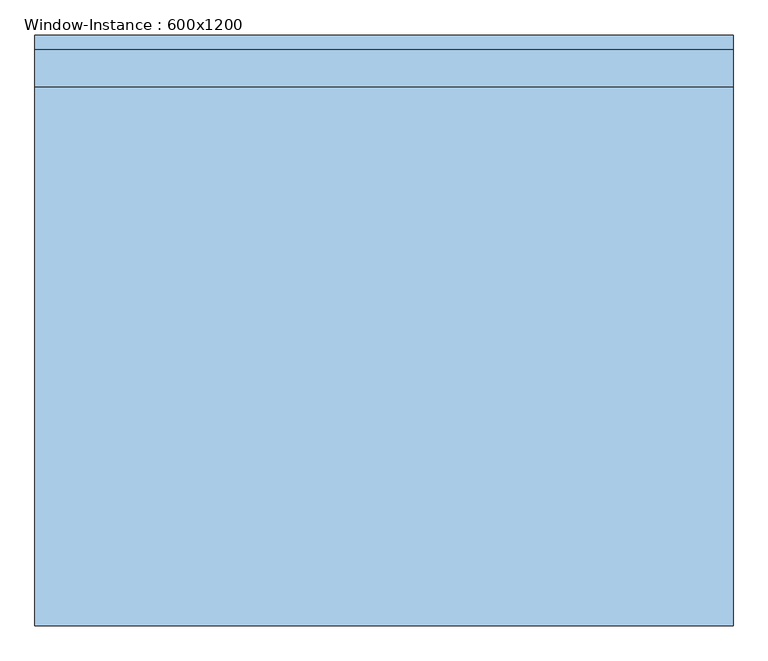
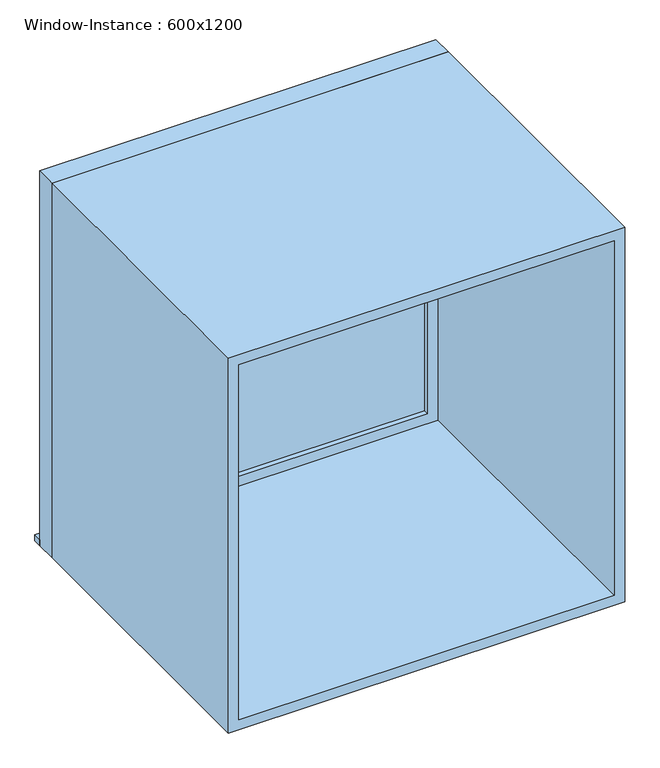
"""IFC4 building model written with IfcOpenShell, lengths in millimetres: window geometry, Window-Instance : 600x1200."""

import ifcopenshell
import ifcopenshell.guid

model = None  # the IFC model being written
_history = None  # IfcOwnerHistory: only IFC2X3 demands one
_inside = {}  # id of a spatial element -> (the spatial element, [elements in it])
_under = {}  # id of a project, library or spatial element -> (it, [spatial elements below it])
_declared = {}  # id of a project -> (the project, [libraries it declares])
_typed = {}  # id of a type object -> (the type object, [elements of that type])
_made_of = {}  # id of a material, layer set ... -> (it, [elements and type objects made of it])


def new_model(schema):
    """Start an empty IFC model of exactly this schema.

    Asked for "IFC4X3", IfcOpenShell would pick the latest addendum, in which some entities
    have other attributes; the version numbers below select the first issue.
    IFC2X3 requires an IfcOwnerHistory on every rooted entity: one is made here for all.
    """
    global model, _history
    if schema == "IFC4X3":
        model = ifcopenshell.file(schema_version=(4, 3, 0, 0))
    else:
        model = ifcopenshell.file(schema=schema)
    _inside.clear()
    _under.clear()
    _declared.clear()
    _typed.clear()
    _made_of.clear()
    _history = None
    if model.schema == "IFC2X3":
        org = make("IfcOrganization", Name="unknown")
        user = make(
            "IfcPersonAndOrganization",
            ThePerson=make("IfcPerson", FamilyName="unknown"),
            TheOrganization=org,
        )
        app = make(
            "IfcApplication",
            ApplicationDeveloper=org,
            Version="unknown",
            ApplicationFullName="unknown",
            ApplicationIdentifier="unknown",
        )
        _history = make(
            "IfcOwnerHistory",
            OwningUser=user,
            OwningApplication=app,
            ChangeAction="ADDED",
            CreationDate=0,
        )
    return model


def make(cls, **values):
    """One entity of the class cls with the attributes given. An attribute that is None is left unset."""
    return model.create_entity(
        cls, **{name: value for name, value in values.items() if value is not None}
    )


def rooted(cls, **values):
    """An entity with a GlobalId (a new one), such as an element, a storey or a relation."""
    return make(cls, GlobalId=ifcopenshell.guid.new(), OwnerHistory=_history, **values)


def si_unit(unit_type, name, prefix=None):
    """IfcSIUnit, for example si_unit("LENGTHUNIT", "METRE", prefix="MILLI")."""
    return make("IfcSIUnit", UnitType=unit_type, Prefix=prefix, Name=name)


def assignment(units):
    """IfcUnitAssignment: the units of a project."""
    return None if units is None else make("IfcUnitAssignment", Units=units)


def point(xyz):
    """IfcCartesianPoint."""
    return None if xyz is None else make("IfcCartesianPoint", Coordinates=xyz)


def direction(xyz):
    """IfcDirection."""
    return None if xyz is None else make("IfcDirection", DirectionRatios=xyz)


def frame(location, z_axis=None, x_axis=None):
    """IfcAxis2Placement3D, a coordinate frame: its origin and axes. An axis left out is left unset."""
    return make(
        "IfcAxis2Placement3D",
        Location=point(location),
        Axis=direction(z_axis),
        RefDirection=direction(x_axis),
    )


def origin():
    """The frame at (0, 0, 0) with its axes left unset."""
    return frame((0.0, 0.0, 0.0))


def place(relative_to, where):
    """IfcLocalPlacement: puts the frame where relative to a parent placement (None: the world)."""
    return make(
        "IfcLocalPlacement", PlacementRelTo=relative_to, RelativePlacement=where
    )


def context(
    kind, dimensions, precision=None, world=None, true_north=None, identifier=None
):
    """IfcGeometricRepresentationContext, for example the 3D "Model" context."""
    return make(
        "IfcGeometricRepresentationContext",
        ContextIdentifier=identifier,
        ContextType=kind,
        CoordinateSpaceDimension=dimensions,
        Precision=precision,
        WorldCoordinateSystem=world,
        TrueNorth=true_north,
    )


def project(units=None, contexts=None):
    """IfcProject with its units and contexts."""
    return rooted(
        "IfcProject",
        Name="project",
        RepresentationContexts=contexts,
        UnitsInContext=assignment(units),
    )


def spatial(cls, under=None, at=None, **own):
    """A site, building, storey or space (cls), placed at a placement, below another one or the project."""
    s = rooted(cls, ObjectPlacement=at, **own)
    if under is not None:
        _under.setdefault(under.id(), (under, []))[1].append(s)
    return s


def polyline(points):
    """IfcPolyline through the points."""
    return make("IfcPolyline", Points=[point(p) for p in points])


def outline(outer, holes=None, kind="AREA"):
    """IfcArbitraryClosedProfileDef: a profile drawn as a closed curve; with holes, ...WithVoids."""
    if holes is None:
        return make("IfcArbitraryClosedProfileDef", ProfileType=kind, OuterCurve=outer)
    return make(
        "IfcArbitraryProfileDefWithVoids",
        ProfileType=kind,
        OuterCurve=outer,
        InnerCurves=holes,
    )


def extrude(swept, where, along, depth):
    """IfcExtrudedAreaSolid: the profile swept, set in the frame where, extruded along a direction by depth."""
    return make(
        "IfcExtrudedAreaSolid",
        SweptArea=swept,
        Position=where,
        ExtrudedDirection=direction(along),
        Depth=depth,
    )


def shape(context_of_items, identifier, shape_type, items):
    """IfcShapeRepresentation: the items that make up one representation, for example the "Body"."""
    return make(
        "IfcShapeRepresentation",
        ContextOfItems=context_of_items,
        RepresentationIdentifier=identifier,
        RepresentationType=shape_type,
        Items=items,
    )


def source(mapping_origin, context_of_items, identifier, shape_type, items):
    """IfcRepresentationMap: a shape defined once, which mapped items show again and again."""
    return make(
        "IfcRepresentationMap",
        MappingOrigin=mapping_origin,
        MappedRepresentation=shape(context_of_items, identifier, shape_type, items),
    )


def transform(
    local_origin,
    x_axis=None,
    y_axis=None,
    z_axis=None,
    scale=None,
    scale2=None,
    scale3=None,
    uniform=True,
):
    """IfcCartesianTransformationOperator3D, or its non-uniform kind. x_axis, y_axis, z_axis: its Axis1, 2, 3."""
    if uniform:
        return make(
            "IfcCartesianTransformationOperator3D",
            Axis1=direction(x_axis),
            Axis2=direction(y_axis),
            LocalOrigin=point(local_origin),
            Scale=scale,
            Axis3=direction(z_axis),
        )
    return make(
        "IfcCartesianTransformationOperator3DnonUniform",
        Axis1=direction(x_axis),
        Axis2=direction(y_axis),
        LocalOrigin=point(local_origin),
        Scale=scale,
        Axis3=direction(z_axis),
        Scale2=scale2,
        Scale3=scale3,
    )


def mapped(mapping_source, mapping_target):
    """IfcMappedItem: shows the shape of a source again, moved by a transform."""
    return make(
        "IfcMappedItem", MappingSource=mapping_source, MappingTarget=mapping_target
    )


def made_of(thing, what):
    """Note that an element or type object is made of a material, layer set ...; save() writes the relation."""
    if what is not None:
        _made_of.setdefault(what.id(), (what, []))[1].append(thing)
    return thing


def element(
    cls,
    number,
    at=None,
    inside=None,
    cuts=None,
    type_object=None,
    material=None,
    context=None,
    identifier="Body",
    shape_type=None,
    held_by="IfcProductDefinitionShape",
    body=None,
    shapes=None,
    **own,
):
    """One element of the class cls, such as IfcWall. Its Tag is "e" and its number.

    at: its placement. inside: the storey or other place that contains it. cuts: it is an
    opening in that element (IfcRelVoidsElement). A single representation is given by context,
    identifier, shape_type and body (its items); several are given by shapes. held_by: the class
    of the entity that holds the representations. save() writes the other relations.
    """
    e = rooted(cls, Tag="e%d" % number, ObjectPlacement=at, **own)
    if body is not None:
        shapes = [shape(context, identifier, shape_type, body)]
    if shapes is not None:
        e.Representation = make(held_by, Representations=shapes)
    if inside is not None:
        _inside.setdefault(inside.id(), (inside, []))[1].append(e)
    if cuts is not None:
        rooted(
            "IfcRelVoidsElement", RelatingBuildingElement=cuts, RelatedOpeningElement=e
        )
    if type_object is not None:
        _typed.setdefault(type_object.id(), (type_object, []))[1].append(e)
    return made_of(e, material)


def aggregate(whole, parts):
    """IfcRelAggregates: a whole, such as a stair, and the parts it consists of."""
    return rooted("IfcRelAggregates", RelatingObject=whole, RelatedObjects=parts)


def save(model, path):
    """Write the relations noted so far, then the file.

    IfcRelAggregates (storeys below a building ...), IfcRelContainedInSpatialStructure (elements
    in a storey), IfcRelDefinesByType, IfcRelAssociatesMaterial and IfcRelDeclares: one each for
    every whole, place, type object, material and project.
    """
    for whole, parts in _under.values():
        aggregate(whole, parts)
    for where, things in _inside.values():
        rooted(
            "IfcRelContainedInSpatialStructure",
            RelatedElements=things,
            RelatingStructure=where,
        )
    for kind, things in _typed.values():
        rooted("IfcRelDefinesByType", RelatedObjects=things, RelatingType=kind)
    for what, things in _made_of.values():
        rooted("IfcRelAssociatesMaterial", RelatedObjects=things, RelatingMaterial=what)
    for by, libraries in _declared.values():
        rooted("IfcRelDeclares", RelatingContext=by, RelatedDefinitions=libraries)
    model.write(path)


def window_instance_600x1200_03e1e92d(model_context):
    return source(origin(), model_context, "Body", "SweptSolid", [
        extrude(outline(polyline([(-638.1, 520.4), (561.9, 520.4), (561.9, 495.0), (-638.1, 495.0), (-638.1, 520.4)])), frame((0.0, 0.0, 900.0), z_axis=(0.0, 0.0, 1.0), x_axis=(1.0, 0.0, 0.0)), (0.0, 0.0, 1.0), 19.05),
        extrude(outline(polyline([(498.4, 446.425), (-574.6, 446.425), (-574.6, 459.125), (498.4, 459.125), (498.4, 446.425)])), frame((0.0, 0.0, 963.5), z_axis=(0.0, 0.0, 1.0), x_axis=(1.0, 0.0, 0.0)), (0.0, 0.0, 1.0), 1073.0),
        extrude(outline(polyline([(2080.95, -619.05), (919.05, -619.05), (919.05, 542.85), (2080.95, 542.85), (2080.95, -619.05)]), holes=[polyline([(2036.5, -574.6), (2036.5, 498.4), (963.5, 498.4), (963.5, -574.6), (2036.5, -574.6)])]), frame((0.0, 430.55, 0.0), z_axis=(0.0, 1.0, 0.0), x_axis=(0.0, 0.0, 1.0)), (0.0, 0.0, 1.0), 44.45),
        extrude(outline(polyline([(2100.0, -638.1), (900.0, -638.1), (900.0, 561.9), (2100.0, 561.9), (2100.0, -638.1)]), holes=[polyline([(2068.25, -606.35), (2068.25, 530.15), (931.75, 530.15), (931.75, -606.35), (2068.25, -606.35)])]), frame((0.0, -495.0, 0.0), z_axis=(0.0, 1.0, 0.0), x_axis=(0.0, 0.0, 1.0)), (0.0, 0.0, 1.0), 925.55),
        extrude(outline(polyline([(2100.0, 561.9), (2100.0, -638.1), (900.0, -638.1), (900.0, 561.9), (2100.0, 561.9)]), holes=[polyline([(2080.95, 542.85), (919.05, 542.85), (919.05, -619.05), (2080.95, -619.05), (2080.95, 542.85)])]), frame((0.0, 430.55, 0.0), z_axis=(0.0, 1.0, 0.0), x_axis=(0.0, 0.0, 1.0)), (0.0, 0.0, 1.0), 64.45),
    ])


if __name__ == "__main__":
    model = new_model("IFC4")
    model_context = context("Model", 3, world=origin())
    ifc_project = project(units=[si_unit("LENGTHUNIT", "METRE", prefix="MILLI")], contexts=[model_context])
    site = spatial("IfcSite", under=ifc_project)
    building = spatial("IfcBuilding", under=site)
    placement = place(None, origin())
    window_instance_600x1200_shape = window_instance_600x1200_03e1e92d(model_context)
    element("IfcWindow", 1, ObjectType="Window-Instance : 600x1200", at=placement, inside=building, context=model_context, shape_type="MappedRepresentation", body=[
        mapped(window_instance_600x1200_shape, transform((0.0, 0.0, 0.0), x_axis=(1.0, 0.0, 0.0), y_axis=(0.0, 1.0, 0.0), z_axis=(0.0, 0.0, 1.0))),
    ])
    save(model, "model.ifc")

# Revit data of these elements
# Type "Window-Instance : 600x1200"
#   Type Mark = "7"
#   Construction Type Id = "GSP4R"
#   Assembly Code = "B2020100"
#   Analytic Construction = "1/8 in Pilkington single glazing"
#   Visual Light Transmittance = 0.9
#   Thermal Resistance (R) = 0.149095 (m²·K)/W
#   Solar Heat Gain Coefficient = 0.86
#   Heat Transfer Coefficient (U) = 6.70716 W/(m²·K)
#   Height [instance default] = 1200 mm
#   Default Sill Height = 900 mm
#   Width [instance default] = 600 mm
#   Window Inset = 20 mm
#   Glass Pane Material = WW-EC-GL-Storefront
#   Sash Material = WW-EC-RGB-White
#   Wall Closure = (empty or 0)
# Element 1 (IfcWindow, "Window-Instance : 600x1200")
#   Width = 1200 mm
#   Materials on its faces: "WW-EC-RGB-White", "WW-EC-GL-Storefront"
# Materials
#   "WW-EC-GL-Storefront": class "Glass", colour RGB 236 240 239, transparency 0.85, Description = "Storefront Glass", Cost = 0
#   "WW-EC-RGB-White": class "Generic", colour RGB 255 255 255, transparency 0, Comments = "If region requests off-white, swith asset color to RGB 231-228-220", Description = "Generic Color", Cost = 0
